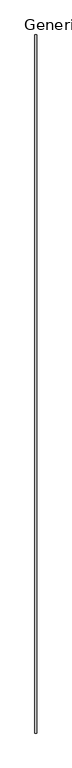
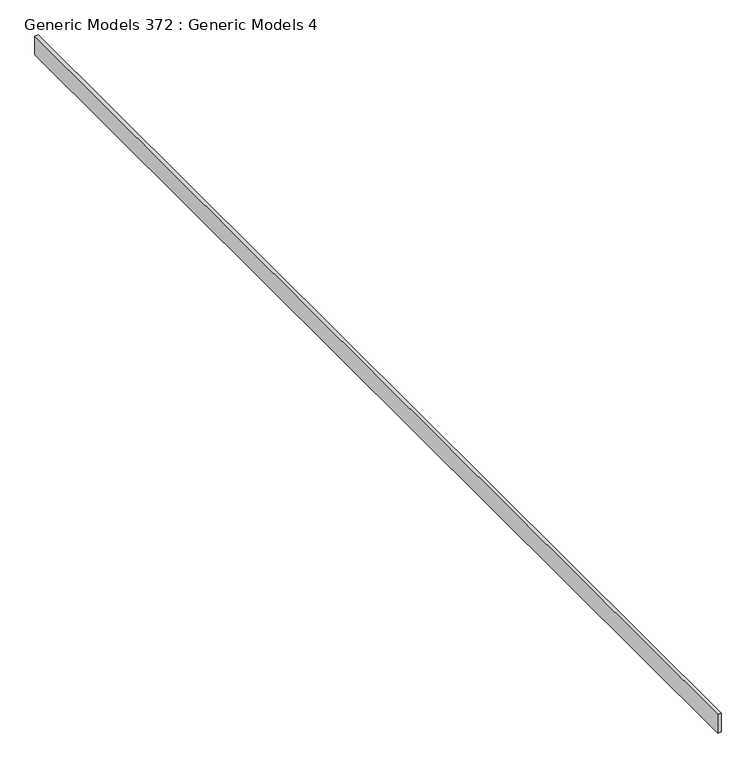
"""IFC4 building model written with IfcOpenShell, lengths in millimetres: proxy geometry, Generic Models 372 : Generic Models 4."""

from ifc_helpers import new_model, si_unit, frame, origin, place, context, project, spatial, polyline, outline, extrude, source, transform, mapped, element, save


def generic_models_372_generic_models_4_70e1e7ac(model_context):
    return source(origin(), model_context, "Body", "SweptSolid", [
        extrude(outline(polyline([(-6337.4736296, -6864.9230338), (-6356.5236296, -6864.9230338), (-6356.5236296, -464.1230338), (-6337.4736296, -464.1230338), (-6337.4736296, -6864.9230338)])), frame((0.0, 0.0, 129006.4087534), z_axis=(0.0, 0.0, 1.0), x_axis=(1.0, 0.0, 0.0)), (0.0, 0.0, 1.0), 107.8244931),
    ])


if __name__ == "__main__":
    model = new_model("IFC4")
    model_context = context("Model", 3, world=origin())
    ifc_project = project(units=[si_unit("LENGTHUNIT", "METRE", prefix="MILLI")], contexts=[model_context])
    site = spatial("IfcSite", under=ifc_project)
    building = spatial("IfcBuilding", under=site)
    placement = place(None, origin())
    generic_models_372_generic_models_4_shape = generic_models_372_generic_models_4_70e1e7ac(model_context)
    element("IfcBuildingElementProxy", 1, Name="Generic Models 372 : Generic Models 4", ObjectType="Generic Models 372 : Generic Models 4", at=placement, inside=building, context=model_context, shape_type="MappedRepresentation", body=[
        mapped(generic_models_372_generic_models_4_shape, transform((0.0, 0.0, 0.0), x_axis=(1.0, 0.0, 0.0), y_axis=(0.0, 1.0, 0.0), z_axis=(0.0, 0.0, 1.0))),
    ])
    save(model, "model.ifc")

# Revit data of these elements
# Element 1 (IfcBuildingElementProxy, "Generic Models 372 : Generic Models 4")
#   Materials on its faces: "_SOLID HARDWOOD STOCK"
# Materials
#   "_SOLID HARDWOOD STOCK": class "Generic", colour RGB 177 130 114, transparency 0, Cost = 0
